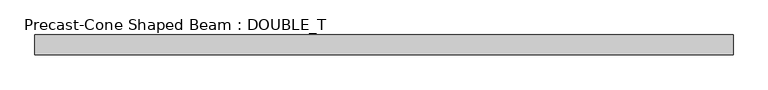
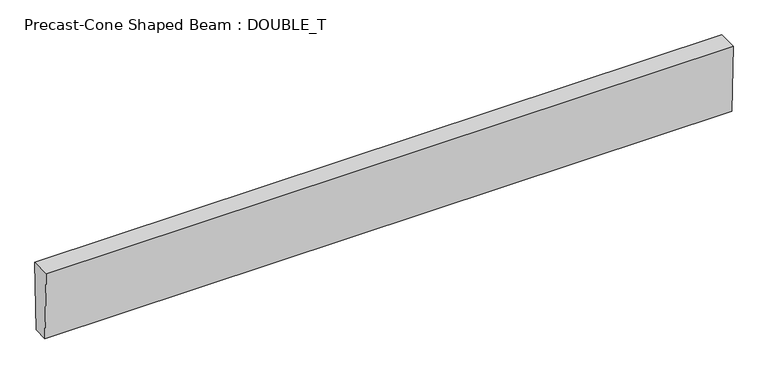
"""IFC4 building model written with IfcOpenShell, lengths in millimetres: beam geometry, Precast-Cone Shaped Beam : DOUBLE_T."""

from ifc_helpers import new_model, si_unit, frame, origin, place, context, project, spatial, polyline, outline, extrude, source, transform, mapped, element, save


def precast_cone_shaped_beam_double_t_ce46092e(model_context):
    return source(origin(), model_context, "Body", "SweptSolid", [
        extrude(outline(polyline([(-50.8, -228.6), (-63.5, 228.6), (63.5, 228.6), (50.8, -228.6), (-50.8, -228.6)])), frame((-2302.66875, 0.0, 0.0), z_axis=(1.0, 0.0, 0.0), x_axis=(0.0, 1.0, 0.0)), (0.0, 0.0, 1.0), 4495.8),
    ])


if __name__ == "__main__":
    model = new_model("IFC4")
    model_context = context("Model", 3, world=origin())
    ifc_project = project(units=[si_unit("LENGTHUNIT", "METRE", prefix="MILLI")], contexts=[model_context])
    site = spatial("IfcSite", under=ifc_project)
    building = spatial("IfcBuilding", under=site)
    placement = place(None, origin())
    precast_cone_shaped_beam_double_t_shape = precast_cone_shaped_beam_double_t_ce46092e(model_context)
    element("IfcBeam", 1, ObjectType="Precast-Cone Shaped Beam : DOUBLE_T", at=placement, inside=building, context=model_context, shape_type="MappedRepresentation", body=[
        mapped(precast_cone_shaped_beam_double_t_shape, transform((0.0, 0.0, 0.0), x_axis=(1.0, 0.0, 0.0), y_axis=(0.0, 1.0, 0.0), z_axis=(0.0, 0.0, 1.0))),
    ])
    save(model, "model.ifc")

# Revit data of these elements
# Type "Precast-Cone Shaped Beam : DOUBLE_T"
#   Top Width = 0' - 5"
#   Tie Rod Weight [instance default] = 30
#   Tie Rod W [instance default] = 0.0660938 kip
#   Single Rebar Weight [instance default] = 50
#   Single Rebar W [instance default] = 0.110156 kip
#   Rebar Grids Weight [instance default] = 100
#   Rebar Grids W [instance default] = 0.220313 kip
#   Depth = 1' - 6"
#   Bottom Width = 0' - 4"
#   Length [instance default] = 5' - 0"
#   Structural Material [instance default] = Concrete, Precast
#   Assembly Code = ""
# Element 1 (IfcBeam, "Precast-Cone Shaped Beam : DOUBLE_T")
#   Length = 14' - 4 11/16"
#   Structural Material = Concrete - Precast Concrete - Normal Weight Concrete - 5 ksi
#   Materials on its faces: "Concrete - Precast Concrete - Normal Weight Concrete - 5 ksi"
# Materials
#   "Concrete, Precast": class "Concrete", colour RGB 198 187 187, transparency 0, Description = "Precast concrete", Cost = 0
#   "Concrete - Precast Concrete - Normal Weight Concrete - 5 ksi": class "Concrete", colour RGB 198 187 187, transparency 0, Cost = 0
